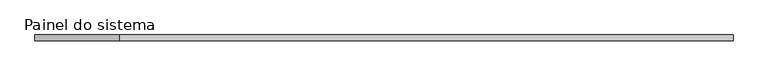
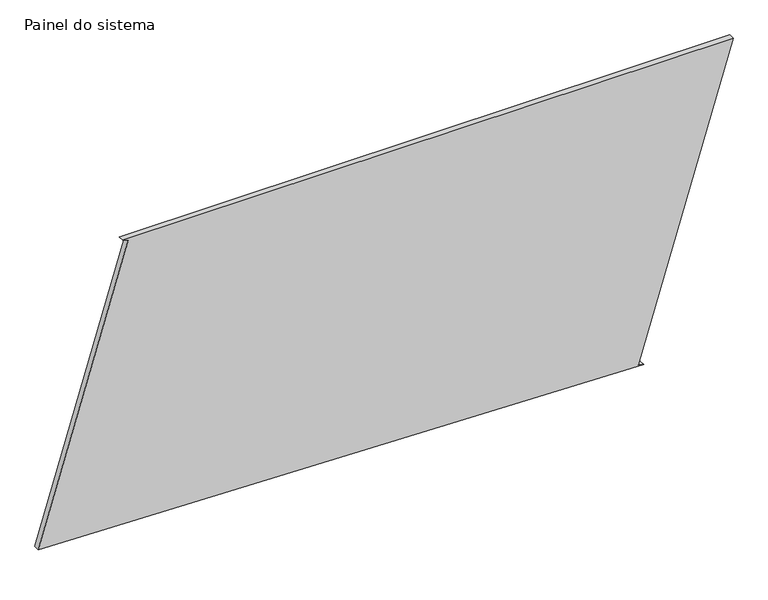
"""IFC4 building model written with IfcOpenShell, lengths in millimetres: plate geometry, Painel do sistema : Envidraçado."""

from ifc_helpers import new_model, si_unit, frame, origin, place, context, project, spatial, polyline, outline, extrude, source, transform, mapped, element, save


def painel_do_sistema_e3572a27(model_context):
    return source(origin(), model_context, "Body", "SweptSolid", [
        extrude(outline(polyline([(0.0, 1125.4886899), (7.2712141, 1101.5694624), (1370.0548184, 1515.842512), (1370.0548184, -1146.8991407), (1362.7836043, -1122.9799132), (70.4313529, -1515.842512), (0.0, 1125.4886899)])), frame((0.0, 24.5, 0.0), z_axis=(0.0, 1.0, 0.0), x_axis=(0.0, 0.0, 1.0)), (0.0, 0.0, 1.0), 25.0),
    ])


if __name__ == "__main__":
    model = new_model("IFC4")
    model_context = context("Model", 3, world=origin())
    ifc_project = project(units=[si_unit("LENGTHUNIT", "METRE", prefix="MILLI")], contexts=[model_context])
    site = spatial("IfcSite", under=ifc_project)
    building = spatial("IfcBuilding", under=site)
    placement = place(None, origin())
    painel_do_sistema_shape = painel_do_sistema_e3572a27(model_context)
    element("IfcPlate", 1, ObjectType="Painel do sistema : Envidraçado", at=placement, inside=building, context=model_context, shape_type="MappedRepresentation", body=[
        mapped(painel_do_sistema_shape, transform((0.0, 0.0, 0.0), x_axis=(1.0, 0.0, 0.0), y_axis=(0.0, 1.0, 0.0), z_axis=(0.0, 0.0, 1.0))),
    ])
    save(model, "model.ifc")

# Revit data of these elements
# Type "Painel do sistema : Envidraçado"
#   Construction Type Id = "GSP4R"
#   Analytic Construction = "Vidraça única Pilkington 1/8 pol"
#   Visual Light Transmittance = 0.9
#   Solar Heat Gain Coefficient = 0.86
#   Heat Transfer Coefficient (U) = 6.7069 W/(m²·K)
# Element 1 (IfcPlate, "Painel do sistema : Envidraçado")
#   Materials on its faces: "Vidro"
# Materials
#   "Vidro": class "Vidro", colour RGB 0 128 192, transparency 0.9, Description = "Vidro de sílica", Cost = 0
